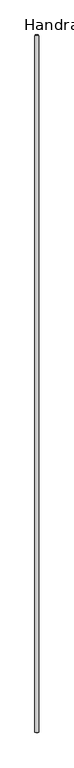
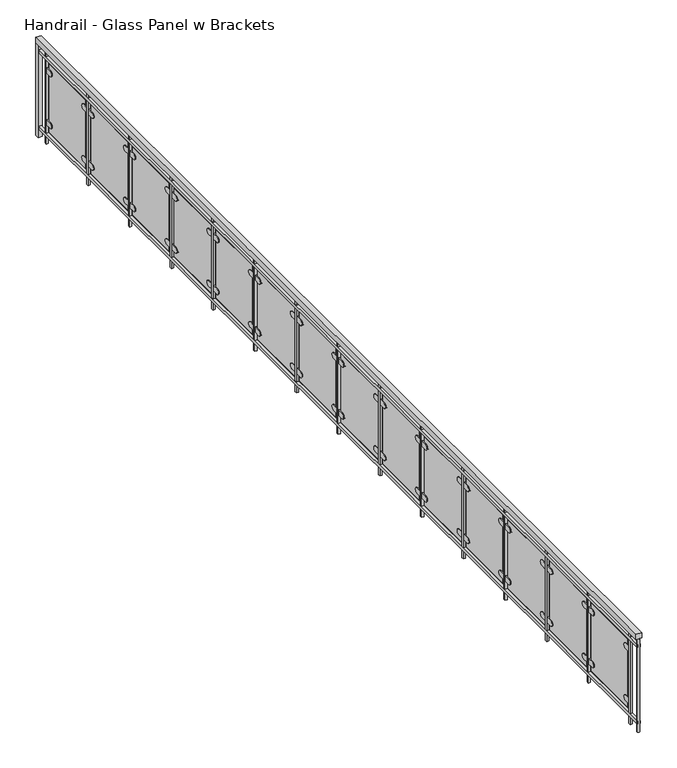
"""IFC4 building model written with IfcOpenShell, lengths in millimetres: railing geometry, Handrail - Glass Panel w Brackets."""

from ifc_helpers import new_model, si_unit, point, frame, frame_2d, origin, origin_with_axes, place, context, project, spatial, polyline, circle_curve, trimmed, segment, composite_curve, outline, extrude, source, transform, mapped, element, save


def handrail_glass_panel_w_brackets_a9dcd3ed(model_context):
    return source(origin(), model_context, "Body", "SweptSolid", [
        extrude(outline(polyline([(-15226.2978678, -5345.4143828), (-15175.4978678, -5345.4143828), (-15175.4978678, -14489.4143828), (-15226.2978678, -14489.4143828), (-15226.2978678, -5345.4143828)])), frame((0.0, 0.0, 863.6), z_axis=(0.0, 0.0, 1.0), x_axis=(1.0, 0.0, 0.0)), (0.0, 0.0, 1.0), 50.8),
        extrude(outline(polyline([(-15213.5978678, -5345.4143828), (-15188.1978678, -5345.4143828), (-15188.1978678, -14489.4143828), (-15213.5978678, -14489.4143828), (-15213.5978678, -5345.4143828)])), frame((0.0, 0.0, 787.4), z_axis=(0.0, 0.0, 1.0), x_axis=(1.0, 0.0, 0.0)), (0.0, 0.0, 1.0), 25.4),
        extrude(outline(polyline([(-15213.5978678, -5345.4143828), (-15188.1978678, -5345.4143828), (-15188.1978678, -14489.4143828), (-15213.5978678, -14489.4143828), (-15213.5978678, -5345.4143828)])), frame((0.0, 0.0, 76.2), z_axis=(0.0, 0.0, 1.0), x_axis=(1.0, 0.0, 0.0)), (0.0, 0.0, 1.0), 25.4),
        extrude(outline(polyline([(-15210.4228678, -14352.8893828), (-15191.3728678, -14352.8893828), (-15191.3728678, -14371.9393828), (-15210.4228678, -14371.9393828), (-15210.4228678, -14352.8893828)])), origin_with_axes(), (0.0, 0.0, 1.0), 863.6),
        extrude(outline(composite_curve([segment(trimmed(circle_curve(frame_2d((-14298.9143828, 685.8)), 25.4), [point((-14298.9143828, 711.2))], [point((-14298.9143828, 660.4))], False, "CARTESIAN"), True, "CONTINUOUS"), segment(polyline([(-14298.9143828, 660.4), (-14349.7143828, 660.4), (-14349.7143828, 711.2), (-14298.9143828, 711.2)]), True, "CONTINUOUS")], self_intersect=False)), frame((-15207.2478678, 0.0, 0.0), z_axis=(1.0, 0.0, 0.0), x_axis=(0.0, 1.0, 0.0)), (0.0, 0.0, 1.0), 19.05),
        extrude(outline(composite_curve([segment(polyline([(-13790.9143828, 711.2), (-13740.1143828, 711.2), (-13740.1143828, 660.4), (-13790.9143828, 660.4)]), True, "CONTINUOUS"), segment(trimmed(circle_curve(frame_2d((-13790.9143828, 685.8)), 25.4), [point((-13790.9143828, 660.4))], [point((-13790.9143828, 711.2))], False, "CARTESIAN"), True, "CONTINUOUS")], self_intersect=False)), frame((-15207.2478678, 0.0, 0.0), z_axis=(1.0, 0.0, 0.0), x_axis=(0.0, 1.0, 0.0)), (0.0, 0.0, 1.0), 19.05),
        extrude(outline(composite_curve([segment(trimmed(circle_curve(frame_2d((-14298.9143828, 203.2)), 25.4), [point((-14298.9143828, 228.6))], [point((-14298.9143828, 177.8))], False, "CARTESIAN"), True, "CONTINUOUS"), segment(polyline([(-14298.9143828, 177.8), (-14349.7143828, 177.8), (-14349.7143828, 228.6), (-14298.9143828, 228.6)]), True, "CONTINUOUS")], self_intersect=False)), frame((-15207.2478678, 0.0, 0.0), z_axis=(1.0, 0.0, 0.0), x_axis=(0.0, 1.0, 0.0)), (0.0, 0.0, 1.0), 19.05),
        extrude(outline(composite_curve([segment(polyline([(-13790.9143828, 228.6), (-13740.1143828, 228.6), (-13740.1143828, 177.8), (-13790.9143828, 177.8)]), True, "CONTINUOUS"), segment(trimmed(circle_curve(frame_2d((-13790.9143828, 203.2)), 25.4), [point((-13790.9143828, 177.8))], [point((-13790.9143828, 228.6))], False, "CARTESIAN"), True, "CONTINUOUS")], self_intersect=False)), frame((-15207.2478678, 0.0, 0.0), z_axis=(1.0, 0.0, 0.0), x_axis=(0.0, 1.0, 0.0)), (0.0, 0.0, 1.0), 19.05),
        extrude(outline(polyline([(-15194.5478678, -13765.5143828), (-15194.5478678, -14324.3143828), (-15200.8978678, -14324.3143828), (-15200.8978678, -13765.5143828), (-15194.5478678, -13765.5143828)])), frame((0.0, 0.0, 127.0), z_axis=(0.0, 0.0, 1.0), x_axis=(1.0, 0.0, 0.0)), (0.0, 0.0, 1.0), 635.0),
        extrude(outline(polyline([(-15210.4228678, -13717.8893828), (-15191.3728678, -13717.8893828), (-15191.3728678, -13736.9393828), (-15210.4228678, -13736.9393828), (-15210.4228678, -13717.8893828)])), origin_with_axes(), (0.0, 0.0, 1.0), 863.6),
        extrude(outline(composite_curve([segment(trimmed(circle_curve(frame_2d((-13663.9143828, 685.8)), 25.4), [point((-13663.9143828, 711.2))], [point((-13663.9143828, 660.4))], False, "CARTESIAN"), True, "CONTINUOUS"), segment(polyline([(-13663.9143828, 660.4), (-13714.7143828, 660.4), (-13714.7143828, 711.2), (-13663.9143828, 711.2)]), True, "CONTINUOUS")], self_intersect=False)), frame((-15207.2478678, 0.0, 0.0), z_axis=(1.0, 0.0, 0.0), x_axis=(0.0, 1.0, 0.0)), (0.0, 0.0, 1.0), 19.05),
        extrude(outline(composite_curve([segment(polyline([(-13155.9143828, 711.2), (-13105.1143828, 711.2), (-13105.1143828, 660.4), (-13155.9143828, 660.4)]), True, "CONTINUOUS"), segment(trimmed(circle_curve(frame_2d((-13155.9143828, 685.8)), 25.4), [point((-13155.9143828, 660.4))], [point((-13155.9143828, 711.2))], False, "CARTESIAN"), True, "CONTINUOUS")], self_intersect=False)), frame((-15207.2478678, 0.0, 0.0), z_axis=(1.0, 0.0, 0.0), x_axis=(0.0, 1.0, 0.0)), (0.0, 0.0, 1.0), 19.05),
        extrude(outline(composite_curve([segment(trimmed(circle_curve(frame_2d((-13663.9143828, 203.2)), 25.4), [point((-13663.9143828, 228.6))], [point((-13663.9143828, 177.8))], False, "CARTESIAN"), True, "CONTINUOUS"), segment(polyline([(-13663.9143828, 177.8), (-13714.7143828, 177.8), (-13714.7143828, 228.6), (-13663.9143828, 228.6)]), True, "CONTINUOUS")], self_intersect=False)), frame((-15207.2478678, 0.0, 0.0), z_axis=(1.0, 0.0, 0.0), x_axis=(0.0, 1.0, 0.0)), (0.0, 0.0, 1.0), 19.05),
        extrude(outline(composite_curve([segment(polyline([(-13155.9143828, 228.6), (-13105.1143828, 228.6), (-13105.1143828, 177.8), (-13155.9143828, 177.8)]), True, "CONTINUOUS"), segment(trimmed(circle_curve(frame_2d((-13155.9143828, 203.2)), 25.4), [point((-13155.9143828, 177.8))], [point((-13155.9143828, 228.6))], False, "CARTESIAN"), True, "CONTINUOUS")], self_intersect=False)), frame((-15207.2478678, 0.0, 0.0), z_axis=(1.0, 0.0, 0.0), x_axis=(0.0, 1.0, 0.0)), (0.0, 0.0, 1.0), 19.05),
        extrude(outline(polyline([(-15194.5478678, -13130.5143828), (-15194.5478678, -13689.3143828), (-15200.8978678, -13689.3143828), (-15200.8978678, -13130.5143828), (-15194.5478678, -13130.5143828)])), frame((0.0, 0.0, 127.0), z_axis=(0.0, 0.0, 1.0), x_axis=(1.0, 0.0, 0.0)), (0.0, 0.0, 1.0), 635.0),
        extrude(outline(polyline([(-15210.4228678, -13082.8893828), (-15191.3728678, -13082.8893828), (-15191.3728678, -13101.9393828), (-15210.4228678, -13101.9393828), (-15210.4228678, -13082.8893828)])), origin_with_axes(), (0.0, 0.0, 1.0), 863.6),
        extrude(outline(composite_curve([segment(trimmed(circle_curve(frame_2d((-13028.9143828, 685.8)), 25.4), [point((-13028.9143828, 711.2))], [point((-13028.9143828, 660.4))], False, "CARTESIAN"), True, "CONTINUOUS"), segment(polyline([(-13028.9143828, 660.4), (-13079.7143828, 660.4), (-13079.7143828, 711.2), (-13028.9143828, 711.2)]), True, "CONTINUOUS")], self_intersect=False)), frame((-15207.2478678, 0.0, 0.0), z_axis=(1.0, 0.0, 0.0), x_axis=(0.0, 1.0, 0.0)), (0.0, 0.0, 1.0), 19.05),
        extrude(outline(composite_curve([segment(polyline([(-12520.9143828, 711.2), (-12470.1143828, 711.2), (-12470.1143828, 660.4), (-12520.9143828, 660.4)]), True, "CONTINUOUS"), segment(trimmed(circle_curve(frame_2d((-12520.9143828, 685.8)), 25.4), [point((-12520.9143828, 660.4))], [point((-12520.9143828, 711.2))], False, "CARTESIAN"), True, "CONTINUOUS")], self_intersect=False)), frame((-15207.2478678, 0.0, 0.0), z_axis=(1.0, 0.0, 0.0), x_axis=(0.0, 1.0, 0.0)), (0.0, 0.0, 1.0), 19.05),
        extrude(outline(composite_curve([segment(trimmed(circle_curve(frame_2d((-13028.9143828, 203.2)), 25.4), [point((-13028.9143828, 228.6))], [point((-13028.9143828, 177.8))], False, "CARTESIAN"), True, "CONTINUOUS"), segment(polyline([(-13028.9143828, 177.8), (-13079.7143828, 177.8), (-13079.7143828, 228.6), (-13028.9143828, 228.6)]), True, "CONTINUOUS")], self_intersect=False)), frame((-15207.2478678, 0.0, 0.0), z_axis=(1.0, 0.0, 0.0), x_axis=(0.0, 1.0, 0.0)), (0.0, 0.0, 1.0), 19.05),
        extrude(outline(composite_curve([segment(polyline([(-12520.9143828, 228.6), (-12470.1143828, 228.6), (-12470.1143828, 177.8), (-12520.9143828, 177.8)]), True, "CONTINUOUS"), segment(trimmed(circle_curve(frame_2d((-12520.9143828, 203.2)), 25.4), [point((-12520.9143828, 177.8))], [point((-12520.9143828, 228.6))], False, "CARTESIAN"), True, "CONTINUOUS")], self_intersect=False)), frame((-15207.2478678, 0.0, 0.0), z_axis=(1.0, 0.0, 0.0), x_axis=(0.0, 1.0, 0.0)), (0.0, 0.0, 1.0), 19.05),
        extrude(outline(polyline([(-15194.5478678, -12495.5143828), (-15194.5478678, -13054.3143828), (-15200.8978678, -13054.3143828), (-15200.8978678, -12495.5143828), (-15194.5478678, -12495.5143828)])), frame((0.0, 0.0, 127.0), z_axis=(0.0, 0.0, 1.0), x_axis=(1.0, 0.0, 0.0)), (0.0, 0.0, 1.0), 635.0),
        extrude(outline(polyline([(-15210.4228678, -12447.8893828), (-15191.3728678, -12447.8893828), (-15191.3728678, -12466.9393828), (-15210.4228678, -12466.9393828), (-15210.4228678, -12447.8893828)])), origin_with_axes(), (0.0, 0.0, 1.0), 863.6),
        extrude(outline(composite_curve([segment(trimmed(circle_curve(frame_2d((-12393.9143828, 685.8)), 25.4), [point((-12393.9143828, 711.2))], [point((-12393.9143828, 660.4))], False, "CARTESIAN"), True, "CONTINUOUS"), segment(polyline([(-12393.9143828, 660.4), (-12444.7143828, 660.4), (-12444.7143828, 711.2), (-12393.9143828, 711.2)]), True, "CONTINUOUS")], self_intersect=False)), frame((-15207.2478678, 0.0, 0.0), z_axis=(1.0, 0.0, 0.0), x_axis=(0.0, 1.0, 0.0)), (0.0, 0.0, 1.0), 19.05),
        extrude(outline(composite_curve([segment(polyline([(-11885.9143828, 711.2), (-11835.1143828, 711.2), (-11835.1143828, 660.4), (-11885.9143828, 660.4)]), True, "CONTINUOUS"), segment(trimmed(circle_curve(frame_2d((-11885.9143828, 685.8)), 25.4), [point((-11885.9143828, 660.4))], [point((-11885.9143828, 711.2))], False, "CARTESIAN"), True, "CONTINUOUS")], self_intersect=False)), frame((-15207.2478678, 0.0, 0.0), z_axis=(1.0, 0.0, 0.0), x_axis=(0.0, 1.0, 0.0)), (0.0, 0.0, 1.0), 19.05),
        extrude(outline(composite_curve([segment(trimmed(circle_curve(frame_2d((-12393.9143828, 203.2)), 25.4), [point((-12393.9143828, 228.6))], [point((-12393.9143828, 177.8))], False, "CARTESIAN"), True, "CONTINUOUS"), segment(polyline([(-12393.9143828, 177.8), (-12444.7143828, 177.8), (-12444.7143828, 228.6), (-12393.9143828, 228.6)]), True, "CONTINUOUS")], self_intersect=False)), frame((-15207.2478678, 0.0, 0.0), z_axis=(1.0, 0.0, 0.0), x_axis=(0.0, 1.0, 0.0)), (0.0, 0.0, 1.0), 19.05),
        extrude(outline(composite_curve([segment(polyline([(-11885.9143828, 228.6), (-11835.1143828, 228.6), (-11835.1143828, 177.8), (-11885.9143828, 177.8)]), True, "CONTINUOUS"), segment(trimmed(circle_curve(frame_2d((-11885.9143828, 203.2)), 25.4), [point((-11885.9143828, 177.8))], [point((-11885.9143828, 228.6))], False, "CARTESIAN"), True, "CONTINUOUS")], self_intersect=False)), frame((-15207.2478678, 0.0, 0.0), z_axis=(1.0, 0.0, 0.0), x_axis=(0.0, 1.0, 0.0)), (0.0, 0.0, 1.0), 19.05),
        extrude(outline(polyline([(-15194.5478678, -11860.5143828), (-15194.5478678, -12419.3143828), (-15200.8978678, -12419.3143828), (-15200.8978678, -11860.5143828), (-15194.5478678, -11860.5143828)])), frame((0.0, 0.0, 127.0), z_axis=(0.0, 0.0, 1.0), x_axis=(1.0, 0.0, 0.0)), (0.0, 0.0, 1.0), 635.0),
        extrude(outline(polyline([(-15210.4228678, -11812.8893828), (-15191.3728678, -11812.8893828), (-15191.3728678, -11831.9393828), (-15210.4228678, -11831.9393828), (-15210.4228678, -11812.8893828)])), origin_with_axes(), (0.0, 0.0, 1.0), 863.6),
        extrude(outline(composite_curve([segment(trimmed(circle_curve(frame_2d((-11758.9143828, 685.8)), 25.4), [point((-11758.9143828, 711.2))], [point((-11758.9143828, 660.4))], False, "CARTESIAN"), True, "CONTINUOUS"), segment(polyline([(-11758.9143828, 660.4), (-11809.7143828, 660.4), (-11809.7143828, 711.2), (-11758.9143828, 711.2)]), True, "CONTINUOUS")], self_intersect=False)), frame((-15207.2478678, 0.0, 0.0), z_axis=(1.0, 0.0, 0.0), x_axis=(0.0, 1.0, 0.0)), (0.0, 0.0, 1.0), 19.05),
        extrude(outline(composite_curve([segment(polyline([(-11250.9143828, 711.2), (-11200.1143828, 711.2), (-11200.1143828, 660.4), (-11250.9143828, 660.4)]), True, "CONTINUOUS"), segment(trimmed(circle_curve(frame_2d((-11250.9143828, 685.8)), 25.4), [point((-11250.9143828, 660.4))], [point((-11250.9143828, 711.2))], False, "CARTESIAN"), True, "CONTINUOUS")], self_intersect=False)), frame((-15207.2478678, 0.0, 0.0), z_axis=(1.0, 0.0, 0.0), x_axis=(0.0, 1.0, 0.0)), (0.0, 0.0, 1.0), 19.05),
        extrude(outline(composite_curve([segment(trimmed(circle_curve(frame_2d((-11758.9143828, 203.2)), 25.4), [point((-11758.9143828, 228.6))], [point((-11758.9143828, 177.8))], False, "CARTESIAN"), True, "CONTINUOUS"), segment(polyline([(-11758.9143828, 177.8), (-11809.7143828, 177.8), (-11809.7143828, 228.6), (-11758.9143828, 228.6)]), True, "CONTINUOUS")], self_intersect=False)), frame((-15207.2478678, 0.0, 0.0), z_axis=(1.0, 0.0, 0.0), x_axis=(0.0, 1.0, 0.0)), (0.0, 0.0, 1.0), 19.05),
        extrude(outline(composite_curve([segment(polyline([(-11250.9143828, 228.6), (-11200.1143828, 228.6), (-11200.1143828, 177.8), (-11250.9143828, 177.8)]), True, "CONTINUOUS"), segment(trimmed(circle_curve(frame_2d((-11250.9143828, 203.2)), 25.4), [point((-11250.9143828, 177.8))], [point((-11250.9143828, 228.6))], False, "CARTESIAN"), True, "CONTINUOUS")], self_intersect=False)), frame((-15207.2478678, 0.0, 0.0), z_axis=(1.0, 0.0, 0.0), x_axis=(0.0, 1.0, 0.0)), (0.0, 0.0, 1.0), 19.05),
        extrude(outline(polyline([(-15194.5478678, -11225.5143828), (-15194.5478678, -11784.3143828), (-15200.8978678, -11784.3143828), (-15200.8978678, -11225.5143828), (-15194.5478678, -11225.5143828)])), frame((0.0, 0.0, 127.0), z_axis=(0.0, 0.0, 1.0), x_axis=(1.0, 0.0, 0.0)), (0.0, 0.0, 1.0), 635.0),
        extrude(outline(polyline([(-15210.4228678, -11177.8893828), (-15191.3728678, -11177.8893828), (-15191.3728678, -11196.9393828), (-15210.4228678, -11196.9393828), (-15210.4228678, -11177.8893828)])), origin_with_axes(), (0.0, 0.0, 1.0), 863.6),
        extrude(outline(composite_curve([segment(trimmed(circle_curve(frame_2d((-11123.9143828, 685.8)), 25.4), [point((-11123.9143828, 711.2))], [point((-11123.9143828, 660.4))], False, "CARTESIAN"), True, "CONTINUOUS"), segment(polyline([(-11123.9143828, 660.4), (-11174.7143828, 660.4), (-11174.7143828, 711.2), (-11123.9143828, 711.2)]), True, "CONTINUOUS")], self_intersect=False)), frame((-15207.2478678, 0.0, 0.0), z_axis=(1.0, 0.0, 0.0), x_axis=(0.0, 1.0, 0.0)), (0.0, 0.0, 1.0), 19.05),
        extrude(outline(composite_curve([segment(polyline([(-10615.9143828, 711.2), (-10565.1143828, 711.2), (-10565.1143828, 660.4), (-10615.9143828, 660.4)]), True, "CONTINUOUS"), segment(trimmed(circle_curve(frame_2d((-10615.9143828, 685.8)), 25.4), [point((-10615.9143828, 660.4))], [point((-10615.9143828, 711.2))], False, "CARTESIAN"), True, "CONTINUOUS")], self_intersect=False)), frame((-15207.2478678, 0.0, 0.0), z_axis=(1.0, 0.0, 0.0), x_axis=(0.0, 1.0, 0.0)), (0.0, 0.0, 1.0), 19.05),
        extrude(outline(composite_curve([segment(trimmed(circle_curve(frame_2d((-11123.9143828, 203.2)), 25.4), [point((-11123.9143828, 228.6))], [point((-11123.9143828, 177.8))], False, "CARTESIAN"), True, "CONTINUOUS"), segment(polyline([(-11123.9143828, 177.8), (-11174.7143828, 177.8), (-11174.7143828, 228.6), (-11123.9143828, 228.6)]), True, "CONTINUOUS")], self_intersect=False)), frame((-15207.2478678, 0.0, 0.0), z_axis=(1.0, 0.0, 0.0), x_axis=(0.0, 1.0, 0.0)), (0.0, 0.0, 1.0), 19.05),
        extrude(outline(composite_curve([segment(polyline([(-10615.9143828, 228.6), (-10565.1143828, 228.6), (-10565.1143828, 177.8), (-10615.9143828, 177.8)]), True, "CONTINUOUS"), segment(trimmed(circle_curve(frame_2d((-10615.9143828, 203.2)), 25.4), [point((-10615.9143828, 177.8))], [point((-10615.9143828, 228.6))], False, "CARTESIAN"), True, "CONTINUOUS")], self_intersect=False)), frame((-15207.2478678, 0.0, 0.0), z_axis=(1.0, 0.0, 0.0), x_axis=(0.0, 1.0, 0.0)), (0.0, 0.0, 1.0), 19.05),
        extrude(outline(polyline([(-15194.5478678, -10590.5143828), (-15194.5478678, -11149.3143828), (-15200.8978678, -11149.3143828), (-15200.8978678, -10590.5143828), (-15194.5478678, -10590.5143828)])), frame((0.0, 0.0, 127.0), z_axis=(0.0, 0.0, 1.0), x_axis=(1.0, 0.0, 0.0)), (0.0, 0.0, 1.0), 635.0),
        extrude(outline(polyline([(-15210.4228678, -10542.8893828), (-15191.3728678, -10542.8893828), (-15191.3728678, -10561.9393828), (-15210.4228678, -10561.9393828), (-15210.4228678, -10542.8893828)])), origin_with_axes(), (0.0, 0.0, 1.0), 863.6),
        extrude(outline(composite_curve([segment(trimmed(circle_curve(frame_2d((-10488.9143828, 685.8)), 25.4), [point((-10488.9143828, 711.2))], [point((-10488.9143828, 660.4))], False, "CARTESIAN"), True, "CONTINUOUS"), segment(polyline([(-10488.9143828, 660.4), (-10539.7143828, 660.4), (-10539.7143828, 711.2), (-10488.9143828, 711.2)]), True, "CONTINUOUS")], self_intersect=False)), frame((-15207.2478678, 0.0, 0.0), z_axis=(1.0, 0.0, 0.0), x_axis=(0.0, 1.0, 0.0)), (0.0, 0.0, 1.0), 19.05),
        extrude(outline(composite_curve([segment(polyline([(-9980.9143828, 711.2), (-9930.1143828, 711.2), (-9930.1143828, 660.4), (-9980.9143828, 660.4)]), True, "CONTINUOUS"), segment(trimmed(circle_curve(frame_2d((-9980.9143828, 685.8)), 25.4), [point((-9980.9143828, 660.4))], [point((-9980.9143828, 711.2))], False, "CARTESIAN"), True, "CONTINUOUS")], self_intersect=False)), frame((-15207.2478678, 0.0, 0.0), z_axis=(1.0, 0.0, 0.0), x_axis=(0.0, 1.0, 0.0)), (0.0, 0.0, 1.0), 19.05),
        extrude(outline(composite_curve([segment(trimmed(circle_curve(frame_2d((-10488.9143828, 203.2)), 25.4), [point((-10488.9143828, 228.6))], [point((-10488.9143828, 177.8))], False, "CARTESIAN"), True, "CONTINUOUS"), segment(polyline([(-10488.9143828, 177.8), (-10539.7143828, 177.8), (-10539.7143828, 228.6), (-10488.9143828, 228.6)]), True, "CONTINUOUS")], self_intersect=False)), frame((-15207.2478678, 0.0, 0.0), z_axis=(1.0, 0.0, 0.0), x_axis=(0.0, 1.0, 0.0)), (0.0, 0.0, 1.0), 19.05),
        extrude(outline(composite_curve([segment(polyline([(-9980.9143828, 228.6), (-9930.1143828, 228.6), (-9930.1143828, 177.8), (-9980.9143828, 177.8)]), True, "CONTINUOUS"), segment(trimmed(circle_curve(frame_2d((-9980.9143828, 203.2)), 25.4), [point((-9980.9143828, 177.8))], [point((-9980.9143828, 228.6))], False, "CARTESIAN"), True, "CONTINUOUS")], self_intersect=False)), frame((-15207.2478678, 0.0, 0.0), z_axis=(1.0, 0.0, 0.0), x_axis=(0.0, 1.0, 0.0)), (0.0, 0.0, 1.0), 19.05),
        extrude(outline(polyline([(-15194.5478678, -9955.5143828), (-15194.5478678, -10514.3143828), (-15200.8978678, -10514.3143828), (-15200.8978678, -9955.5143828), (-15194.5478678, -9955.5143828)])), frame((0.0, 0.0, 127.0), z_axis=(0.0, 0.0, 1.0), x_axis=(1.0, 0.0, 0.0)), (0.0, 0.0, 1.0), 635.0),
        extrude(outline(polyline([(-15210.4228678, -9907.8893828), (-15191.3728678, -9907.8893828), (-15191.3728678, -9926.9393828), (-15210.4228678, -9926.9393828), (-15210.4228678, -9907.8893828)])), origin_with_axes(), (0.0, 0.0, 1.0), 863.6),
        extrude(outline(composite_curve([segment(trimmed(circle_curve(frame_2d((-9853.9143828, 685.8)), 25.4), [point((-9853.9143828, 711.2))], [point((-9853.9143828, 660.4))], False, "CARTESIAN"), True, "CONTINUOUS"), segment(polyline([(-9853.9143828, 660.4), (-9904.7143828, 660.4), (-9904.7143828, 711.2), (-9853.9143828, 711.2)]), True, "CONTINUOUS")], self_intersect=False)), frame((-15207.2478678, 0.0, 0.0), z_axis=(1.0, 0.0, 0.0), x_axis=(0.0, 1.0, 0.0)), (0.0, 0.0, 1.0), 19.05),
        extrude(outline(composite_curve([segment(polyline([(-9345.9143828, 711.2), (-9295.1143828, 711.2), (-9295.1143828, 660.4), (-9345.9143828, 660.4)]), True, "CONTINUOUS"), segment(trimmed(circle_curve(frame_2d((-9345.9143828, 685.8)), 25.4), [point((-9345.9143828, 660.4))], [point((-9345.9143828, 711.2))], False, "CARTESIAN"), True, "CONTINUOUS")], self_intersect=False)), frame((-15207.2478678, 0.0, 0.0), z_axis=(1.0, 0.0, 0.0), x_axis=(0.0, 1.0, 0.0)), (0.0, 0.0, 1.0), 19.05),
        extrude(outline(composite_curve([segment(trimmed(circle_curve(frame_2d((-9853.9143828, 203.2)), 25.4), [point((-9853.9143828, 228.6))], [point((-9853.9143828, 177.8))], False, "CARTESIAN"), True, "CONTINUOUS"), segment(polyline([(-9853.9143828, 177.8), (-9904.7143828, 177.8), (-9904.7143828, 228.6), (-9853.9143828, 228.6)]), True, "CONTINUOUS")], self_intersect=False)), frame((-15207.2478678, 0.0, 0.0), z_axis=(1.0, 0.0, 0.0), x_axis=(0.0, 1.0, 0.0)), (0.0, 0.0, 1.0), 19.05),
        extrude(outline(composite_curve([segment(polyline([(-9345.9143828, 228.6), (-9295.1143828, 228.6), (-9295.1143828, 177.8), (-9345.9143828, 177.8)]), True, "CONTINUOUS"), segment(trimmed(circle_curve(frame_2d((-9345.9143828, 203.2)), 25.4), [point((-9345.9143828, 177.8))], [point((-9345.9143828, 228.6))], False, "CARTESIAN"), True, "CONTINUOUS")], self_intersect=False)), frame((-15207.2478678, 0.0, 0.0), z_axis=(1.0, 0.0, 0.0), x_axis=(0.0, 1.0, 0.0)), (0.0, 0.0, 1.0), 19.05),
        extrude(outline(polyline([(-15194.5478678, -9320.5143828), (-15194.5478678, -9879.3143828), (-15200.8978678, -9879.3143828), (-15200.8978678, -9320.5143828), (-15194.5478678, -9320.5143828)])), frame((0.0, 0.0, 127.0), z_axis=(0.0, 0.0, 1.0), x_axis=(1.0, 0.0, 0.0)), (0.0, 0.0, 1.0), 635.0),
        extrude(outline(polyline([(-15210.4228678, -9272.8893828), (-15191.3728678, -9272.8893828), (-15191.3728678, -9291.9393828), (-15210.4228678, -9291.9393828), (-15210.4228678, -9272.8893828)])), origin_with_axes(), (0.0, 0.0, 1.0), 863.6),
        extrude(outline(composite_curve([segment(trimmed(circle_curve(frame_2d((-9218.9143828, 685.8)), 25.4), [point((-9218.9143828, 711.2))], [point((-9218.9143828, 660.4))], False, "CARTESIAN"), True, "CONTINUOUS"), segment(polyline([(-9218.9143828, 660.4), (-9269.7143828, 660.4), (-9269.7143828, 711.2), (-9218.9143828, 711.2)]), True, "CONTINUOUS")], self_intersect=False)), frame((-15207.2478678, 0.0, 0.0), z_axis=(1.0, 0.0, 0.0), x_axis=(0.0, 1.0, 0.0)), (0.0, 0.0, 1.0), 19.05),
        extrude(outline(composite_curve([segment(polyline([(-8710.9143828, 711.2), (-8660.1143828, 711.2), (-8660.1143828, 660.4), (-8710.9143828, 660.4)]), True, "CONTINUOUS"), segment(trimmed(circle_curve(frame_2d((-8710.9143828, 685.8)), 25.4), [point((-8710.9143828, 660.4))], [point((-8710.9143828, 711.2))], False, "CARTESIAN"), True, "CONTINUOUS")], self_intersect=False)), frame((-15207.2478678, 0.0, 0.0), z_axis=(1.0, 0.0, 0.0), x_axis=(0.0, 1.0, 0.0)), (0.0, 0.0, 1.0), 19.05),
        extrude(outline(composite_curve([segment(trimmed(circle_curve(frame_2d((-9218.9143828, 203.2)), 25.4), [point((-9218.9143828, 228.6))], [point((-9218.9143828, 177.8))], False, "CARTESIAN"), True, "CONTINUOUS"), segment(polyline([(-9218.9143828, 177.8), (-9269.7143828, 177.8), (-9269.7143828, 228.6), (-9218.9143828, 228.6)]), True, "CONTINUOUS")], self_intersect=False)), frame((-15207.2478678, 0.0, 0.0), z_axis=(1.0, 0.0, 0.0), x_axis=(0.0, 1.0, 0.0)), (0.0, 0.0, 1.0), 19.05),
        extrude(outline(composite_curve([segment(polyline([(-8710.9143828, 228.6), (-8660.1143828, 228.6), (-8660.1143828, 177.8), (-8710.9143828, 177.8)]), True, "CONTINUOUS"), segment(trimmed(circle_curve(frame_2d((-8710.9143828, 203.2)), 25.4), [point((-8710.9143828, 177.8))], [point((-8710.9143828, 228.6))], False, "CARTESIAN"), True, "CONTINUOUS")], self_intersect=False)), frame((-15207.2478678, 0.0, 0.0), z_axis=(1.0, 0.0, 0.0), x_axis=(0.0, 1.0, 0.0)), (0.0, 0.0, 1.0), 19.05),
        extrude(outline(polyline([(-15194.5478678, -8685.5143828), (-15194.5478678, -9244.3143828), (-15200.8978678, -9244.3143828), (-15200.8978678, -8685.5143828), (-15194.5478678, -8685.5143828)])), frame((0.0, 0.0, 127.0), z_axis=(0.0, 0.0, 1.0), x_axis=(1.0, 0.0, 0.0)), (0.0, 0.0, 1.0), 635.0),
        extrude(outline(polyline([(-15210.4228678, -8637.8893828), (-15191.3728678, -8637.8893828), (-15191.3728678, -8656.9393828), (-15210.4228678, -8656.9393828), (-15210.4228678, -8637.8893828)])), origin_with_axes(), (0.0, 0.0, 1.0), 863.6),
        extrude(outline(composite_curve([segment(trimmed(circle_curve(frame_2d((-8583.9143828, 685.8)), 25.4), [point((-8583.9143828, 711.2))], [point((-8583.9143828, 660.4))], False, "CARTESIAN"), True, "CONTINUOUS"), segment(polyline([(-8583.9143828, 660.4), (-8634.7143828, 660.4), (-8634.7143828, 711.2), (-8583.9143828, 711.2)]), True, "CONTINUOUS")], self_intersect=False)), frame((-15207.2478678, 0.0, 0.0), z_axis=(1.0, 0.0, 0.0), x_axis=(0.0, 1.0, 0.0)), (0.0, 0.0, 1.0), 19.05),
        extrude(outline(composite_curve([segment(polyline([(-8075.9143828, 711.2), (-8025.1143828, 711.2), (-8025.1143828, 660.4), (-8075.9143828, 660.4)]), True, "CONTINUOUS"), segment(trimmed(circle_curve(frame_2d((-8075.9143828, 685.8)), 25.4), [point((-8075.9143828, 660.4))], [point((-8075.9143828, 711.2))], False, "CARTESIAN"), True, "CONTINUOUS")], self_intersect=False)), frame((-15207.2478678, 0.0, 0.0), z_axis=(1.0, 0.0, 0.0), x_axis=(0.0, 1.0, 0.0)), (0.0, 0.0, 1.0), 19.05),
        extrude(outline(composite_curve([segment(trimmed(circle_curve(frame_2d((-8583.9143828, 203.2)), 25.4), [point((-8583.9143828, 228.6))], [point((-8583.9143828, 177.8))], False, "CARTESIAN"), True, "CONTINUOUS"), segment(polyline([(-8583.9143828, 177.8), (-8634.7143828, 177.8), (-8634.7143828, 228.6), (-8583.9143828, 228.6)]), True, "CONTINUOUS")], self_intersect=False)), frame((-15207.2478678, 0.0, 0.0), z_axis=(1.0, 0.0, 0.0), x_axis=(0.0, 1.0, 0.0)), (0.0, 0.0, 1.0), 19.05),
        extrude(outline(composite_curve([segment(polyline([(-8075.9143828, 228.6), (-8025.1143828, 228.6), (-8025.1143828, 177.8), (-8075.9143828, 177.8)]), True, "CONTINUOUS"), segment(trimmed(circle_curve(frame_2d((-8075.9143828, 203.2)), 25.4), [point((-8075.9143828, 177.8))], [point((-8075.9143828, 228.6))], False, "CARTESIAN"), True, "CONTINUOUS")], self_intersect=False)), frame((-15207.2478678, 0.0, 0.0), z_axis=(1.0, 0.0, 0.0), x_axis=(0.0, 1.0, 0.0)), (0.0, 0.0, 1.0), 19.05),
        extrude(outline(polyline([(-15194.5478678, -8050.5143828), (-15194.5478678, -8609.3143828), (-15200.8978678, -8609.3143828), (-15200.8978678, -8050.5143828), (-15194.5478678, -8050.5143828)])), frame((0.0, 0.0, 127.0), z_axis=(0.0, 0.0, 1.0), x_axis=(1.0, 0.0, 0.0)), (0.0, 0.0, 1.0), 635.0),
        extrude(outline(polyline([(-15210.4228678, -8002.8893828), (-15191.3728678, -8002.8893828), (-15191.3728678, -8021.9393828), (-15210.4228678, -8021.9393828), (-15210.4228678, -8002.8893828)])), origin_with_axes(), (0.0, 0.0, 1.0), 863.6),
        extrude(outline(composite_curve([segment(trimmed(circle_curve(frame_2d((-7948.9143828, 685.8)), 25.4), [point((-7948.9143828, 711.2))], [point((-7948.9143828, 660.4))], False, "CARTESIAN"), True, "CONTINUOUS"), segment(polyline([(-7948.9143828, 660.4), (-7999.7143828, 660.4), (-7999.7143828, 711.2), (-7948.9143828, 711.2)]), True, "CONTINUOUS")], self_intersect=False)), frame((-15207.2478678, 0.0, 0.0), z_axis=(1.0, 0.0, 0.0), x_axis=(0.0, 1.0, 0.0)), (0.0, 0.0, 1.0), 19.05),
        extrude(outline(composite_curve([segment(polyline([(-7440.9143828, 711.2), (-7390.1143828, 711.2), (-7390.1143828, 660.4), (-7440.9143828, 660.4)]), True, "CONTINUOUS"), segment(trimmed(circle_curve(frame_2d((-7440.9143828, 685.8)), 25.4), [point((-7440.9143828, 660.4))], [point((-7440.9143828, 711.2))], False, "CARTESIAN"), True, "CONTINUOUS")], self_intersect=False)), frame((-15207.2478678, 0.0, 0.0), z_axis=(1.0, 0.0, 0.0), x_axis=(0.0, 1.0, 0.0)), (0.0, 0.0, 1.0), 19.05),
        extrude(outline(composite_curve([segment(trimmed(circle_curve(frame_2d((-7948.9143828, 203.2)), 25.4), [point((-7948.9143828, 228.6))], [point((-7948.9143828, 177.8))], False, "CARTESIAN"), True, "CONTINUOUS"), segment(polyline([(-7948.9143828, 177.8), (-7999.7143828, 177.8), (-7999.7143828, 228.6), (-7948.9143828, 228.6)]), True, "CONTINUOUS")], self_intersect=False)), frame((-15207.2478678, 0.0, 0.0), z_axis=(1.0, 0.0, 0.0), x_axis=(0.0, 1.0, 0.0)), (0.0, 0.0, 1.0), 19.05),
        extrude(outline(composite_curve([segment(polyline([(-7440.9143828, 228.6), (-7390.1143828, 228.6), (-7390.1143828, 177.8), (-7440.9143828, 177.8)]), True, "CONTINUOUS"), segment(trimmed(circle_curve(frame_2d((-7440.9143828, 203.2)), 25.4), [point((-7440.9143828, 177.8))], [point((-7440.9143828, 228.6))], False, "CARTESIAN"), True, "CONTINUOUS")], self_intersect=False)), frame((-15207.2478678, 0.0, 0.0), z_axis=(1.0, 0.0, 0.0), x_axis=(0.0, 1.0, 0.0)), (0.0, 0.0, 1.0), 19.05),
        extrude(outline(polyline([(-15194.5478678, -7415.5143828), (-15194.5478678, -7974.3143828), (-15200.8978678, -7974.3143828), (-15200.8978678, -7415.5143828), (-15194.5478678, -7415.5143828)])), frame((0.0, 0.0, 127.0), z_axis=(0.0, 0.0, 1.0), x_axis=(1.0, 0.0, 0.0)), (0.0, 0.0, 1.0), 635.0),
        extrude(outline(polyline([(-15210.4228678, -7367.8893828), (-15191.3728678, -7367.8893828), (-15191.3728678, -7386.9393828), (-15210.4228678, -7386.9393828), (-15210.4228678, -7367.8893828)])), origin_with_axes(), (0.0, 0.0, 1.0), 863.6),
        extrude(outline(composite_curve([segment(trimmed(circle_curve(frame_2d((-7313.9143828, 685.8)), 25.4), [point((-7313.9143828, 711.2))], [point((-7313.9143828, 660.4))], False, "CARTESIAN"), True, "CONTINUOUS"), segment(polyline([(-7313.9143828, 660.4), (-7364.7143828, 660.4), (-7364.7143828, 711.2), (-7313.9143828, 711.2)]), True, "CONTINUOUS")], self_intersect=False)), frame((-15207.2478678, 0.0, 0.0), z_axis=(1.0, 0.0, 0.0), x_axis=(0.0, 1.0, 0.0)), (0.0, 0.0, 1.0), 19.05),
        extrude(outline(composite_curve([segment(polyline([(-6805.9143828, 711.2), (-6755.1143828, 711.2), (-6755.1143828, 660.4), (-6805.9143828, 660.4)]), True, "CONTINUOUS"), segment(trimmed(circle_curve(frame_2d((-6805.9143828, 685.8)), 25.4), [point((-6805.9143828, 660.4))], [point((-6805.9143828, 711.2))], False, "CARTESIAN"), True, "CONTINUOUS")], self_intersect=False)), frame((-15207.2478678, 0.0, 0.0), z_axis=(1.0, 0.0, 0.0), x_axis=(0.0, 1.0, 0.0)), (0.0, 0.0, 1.0), 19.05),
        extrude(outline(composite_curve([segment(trimmed(circle_curve(frame_2d((-7313.9143828, 203.2)), 25.4), [point((-7313.9143828, 228.6))], [point((-7313.9143828, 177.8))], False, "CARTESIAN"), True, "CONTINUOUS"), segment(polyline([(-7313.9143828, 177.8), (-7364.7143828, 177.8), (-7364.7143828, 228.6), (-7313.9143828, 228.6)]), True, "CONTINUOUS")], self_intersect=False)), frame((-15207.2478678, 0.0, 0.0), z_axis=(1.0, 0.0, 0.0), x_axis=(0.0, 1.0, 0.0)), (0.0, 0.0, 1.0), 19.05),
        extrude(outline(composite_curve([segment(polyline([(-6805.9143828, 228.6), (-6755.1143828, 228.6), (-6755.1143828, 177.8), (-6805.9143828, 177.8)]), True, "CONTINUOUS"), segment(trimmed(circle_curve(frame_2d((-6805.9143828, 203.2)), 25.4), [point((-6805.9143828, 177.8))], [point((-6805.9143828, 228.6))], False, "CARTESIAN"), True, "CONTINUOUS")], self_intersect=False)), frame((-15207.2478678, 0.0, 0.0), z_axis=(1.0, 0.0, 0.0), x_axis=(0.0, 1.0, 0.0)), (0.0, 0.0, 1.0), 19.05),
        extrude(outline(polyline([(-15194.5478678, -6780.5143828), (-15194.5478678, -7339.3143828), (-15200.8978678, -7339.3143828), (-15200.8978678, -6780.5143828), (-15194.5478678, -6780.5143828)])), frame((0.0, 0.0, 127.0), z_axis=(0.0, 0.0, 1.0), x_axis=(1.0, 0.0, 0.0)), (0.0, 0.0, 1.0), 635.0),
        extrude(outline(polyline([(-15210.4228678, -6732.8893828), (-15191.3728678, -6732.8893828), (-15191.3728678, -6751.9393828), (-15210.4228678, -6751.9393828), (-15210.4228678, -6732.8893828)])), origin_with_axes(), (0.0, 0.0, 1.0), 863.6),
        extrude(outline(composite_curve([segment(trimmed(circle_curve(frame_2d((-6678.9143828, 685.8)), 25.4), [point((-6678.9143828, 711.2))], [point((-6678.9143828, 660.4))], False, "CARTESIAN"), True, "CONTINUOUS"), segment(polyline([(-6678.9143828, 660.4), (-6729.7143828, 660.4), (-6729.7143828, 711.2), (-6678.9143828, 711.2)]), True, "CONTINUOUS")], self_intersect=False)), frame((-15207.2478678, 0.0, 0.0), z_axis=(1.0, 0.0, 0.0), x_axis=(0.0, 1.0, 0.0)), (0.0, 0.0, 1.0), 19.05),
        extrude(outline(composite_curve([segment(polyline([(-6170.9143828, 711.2), (-6120.1143828, 711.2), (-6120.1143828, 660.4), (-6170.9143828, 660.4)]), True, "CONTINUOUS"), segment(trimmed(circle_curve(frame_2d((-6170.9143828, 685.8)), 25.4), [point((-6170.9143828, 660.4))], [point((-6170.9143828, 711.2))], False, "CARTESIAN"), True, "CONTINUOUS")], self_intersect=False)), frame((-15207.2478678, 0.0, 0.0), z_axis=(1.0, 0.0, 0.0), x_axis=(0.0, 1.0, 0.0)), (0.0, 0.0, 1.0), 19.05),
        extrude(outline(composite_curve([segment(trimmed(circle_curve(frame_2d((-6678.9143828, 203.2)), 25.4), [point((-6678.9143828, 228.6))], [point((-6678.9143828, 177.8))], False, "CARTESIAN"), True, "CONTINUOUS"), segment(polyline([(-6678.9143828, 177.8), (-6729.7143828, 177.8), (-6729.7143828, 228.6), (-6678.9143828, 228.6)]), True, "CONTINUOUS")], self_intersect=False)), frame((-15207.2478678, 0.0, 0.0), z_axis=(1.0, 0.0, 0.0), x_axis=(0.0, 1.0, 0.0)), (0.0, 0.0, 1.0), 19.05),
        extrude(outline(composite_curve([segment(polyline([(-6170.9143828, 228.6), (-6120.1143828, 228.6), (-6120.1143828, 177.8), (-6170.9143828, 177.8)]), True, "CONTINUOUS"), segment(trimmed(circle_curve(frame_2d((-6170.9143828, 203.2)), 25.4), [point((-6170.9143828, 177.8))], [point((-6170.9143828, 228.6))], False, "CARTESIAN"), True, "CONTINUOUS")], self_intersect=False)), frame((-15207.2478678, 0.0, 0.0), z_axis=(1.0, 0.0, 0.0), x_axis=(0.0, 1.0, 0.0)), (0.0, 0.0, 1.0), 19.05),
        extrude(outline(polyline([(-15194.5478678, -6145.5143828), (-15194.5478678, -6704.3143828), (-15200.8978678, -6704.3143828), (-15200.8978678, -6145.5143828), (-15194.5478678, -6145.5143828)])), frame((0.0, 0.0, 127.0), z_axis=(0.0, 0.0, 1.0), x_axis=(1.0, 0.0, 0.0)), (0.0, 0.0, 1.0), 635.0),
        extrude(outline(polyline([(-15210.4228678, -6097.8893828), (-15191.3728678, -6097.8893828), (-15191.3728678, -6116.9393828), (-15210.4228678, -6116.9393828), (-15210.4228678, -6097.8893828)])), origin_with_axes(), (0.0, 0.0, 1.0), 863.6),
        extrude(outline(composite_curve([segment(trimmed(circle_curve(frame_2d((-6043.9143828, 685.8)), 25.4), [point((-6043.9143828, 711.2))], [point((-6043.9143828, 660.4))], False, "CARTESIAN"), True, "CONTINUOUS"), segment(polyline([(-6043.9143828, 660.4), (-6094.7143828, 660.4), (-6094.7143828, 711.2), (-6043.9143828, 711.2)]), True, "CONTINUOUS")], self_intersect=False)), frame((-15207.2478678, 0.0, 0.0), z_axis=(1.0, 0.0, 0.0), x_axis=(0.0, 1.0, 0.0)), (0.0, 0.0, 1.0), 19.05),
        extrude(outline(composite_curve([segment(polyline([(-5535.9143828, 711.2), (-5485.1143828, 711.2), (-5485.1143828, 660.4), (-5535.9143828, 660.4)]), True, "CONTINUOUS"), segment(trimmed(circle_curve(frame_2d((-5535.9143828, 685.8)), 25.4), [point((-5535.9143828, 660.4))], [point((-5535.9143828, 711.2))], False, "CARTESIAN"), True, "CONTINUOUS")], self_intersect=False)), frame((-15207.2478678, 0.0, 0.0), z_axis=(1.0, 0.0, 0.0), x_axis=(0.0, 1.0, 0.0)), (0.0, 0.0, 1.0), 19.05),
        extrude(outline(composite_curve([segment(trimmed(circle_curve(frame_2d((-6043.9143828, 203.2)), 25.4), [point((-6043.9143828, 228.6))], [point((-6043.9143828, 177.8))], False, "CARTESIAN"), True, "CONTINUOUS"), segment(polyline([(-6043.9143828, 177.8), (-6094.7143828, 177.8), (-6094.7143828, 228.6), (-6043.9143828, 228.6)]), True, "CONTINUOUS")], self_intersect=False)), frame((-15207.2478678, 0.0, 0.0), z_axis=(1.0, 0.0, 0.0), x_axis=(0.0, 1.0, 0.0)), (0.0, 0.0, 1.0), 19.05),
        extrude(outline(composite_curve([segment(polyline([(-5535.9143828, 228.6), (-5485.1143828, 228.6), (-5485.1143828, 177.8), (-5535.9143828, 177.8)]), True, "CONTINUOUS"), segment(trimmed(circle_curve(frame_2d((-5535.9143828, 203.2)), 25.4), [point((-5535.9143828, 177.8))], [point((-5535.9143828, 228.6))], False, "CARTESIAN"), True, "CONTINUOUS")], self_intersect=False)), frame((-15207.2478678, 0.0, 0.0), z_axis=(1.0, 0.0, 0.0), x_axis=(0.0, 1.0, 0.0)), (0.0, 0.0, 1.0), 19.05),
        extrude(outline(polyline([(-15194.5478678, -5510.5143828), (-15194.5478678, -6069.3143828), (-15200.8978678, -6069.3143828), (-15200.8978678, -5510.5143828), (-15194.5478678, -5510.5143828)])), frame((0.0, 0.0, 127.0), z_axis=(0.0, 0.0, 1.0), x_axis=(1.0, 0.0, 0.0)), (0.0, 0.0, 1.0), 635.0),
        extrude(outline(polyline([(-15210.4228678, -5462.8893828), (-15191.3728678, -5462.8893828), (-15191.3728678, -5481.9393828), (-15210.4228678, -5481.9393828), (-15210.4228678, -5462.8893828)])), origin_with_axes(), (0.0, 0.0, 1.0), 863.6),
        extrude(outline(composite_curve([segment(trimmed(circle_curve(frame_2d((-15200.8978678, -14479.8893828)), 12.7), [point((-15188.1978678, -14479.8893828))], [point((-15213.5978678, -14479.8893828))], False, "CARTESIAN"), True, "CONTINUOUS"), segment(trimmed(circle_curve(frame_2d((-15200.8978678, -14479.8893828)), 12.7), [point((-15213.5978678, -14479.8893828))], [point((-15188.1978678, -14479.8893828))], False, "CARTESIAN"), True, "CONTINUOUS")], self_intersect=False)), origin_with_axes(), (0.0, 0.0, 1.0), 863.6),
        extrude(outline(polyline([(-15219.9478678, -5335.8893828), (-15181.8478678, -5335.8893828), (-15181.8478678, -5373.9893828), (-15219.9478678, -5373.9893828), (-15219.9478678, -5335.8893828)])), origin_with_axes(), (0.0, 0.0, 1.0), 863.6),
    ])


if __name__ == "__main__":
    model = new_model("IFC4")
    model_context = context("Model", 3, world=origin())
    ifc_project = project(units=[si_unit("LENGTHUNIT", "METRE", prefix="MILLI")], contexts=[model_context])
    site = spatial("IfcSite", under=ifc_project)
    building = spatial("IfcBuilding", under=site)
    placement = place(None, origin())
    handrail_glass_panel_w_brackets_shape = handrail_glass_panel_w_brackets_a9dcd3ed(model_context)
    element("IfcRailing", 1, ObjectType="Handrail - Glass Panel w Brackets", at=placement, inside=building, context=model_context, shape_type="MappedRepresentation", body=[
        mapped(handrail_glass_panel_w_brackets_shape, transform((0.0, 0.0, 0.0), x_axis=(1.0, 0.0, 0.0), y_axis=(0.0, 1.0, 0.0), z_axis=(0.0, 0.0, 1.0))),
    ])
    save(model, "model.ifc")

# Revit data of these elements
# Element 1 (IfcRailing, "Handrail - Glass Panel w Brackets")
#   Materials on its faces: "Glass"
# Materials
#   "Glass": class "Unassigned", colour RGB 0 128 192, transparency 0.75
